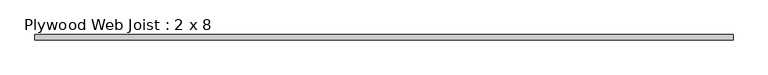
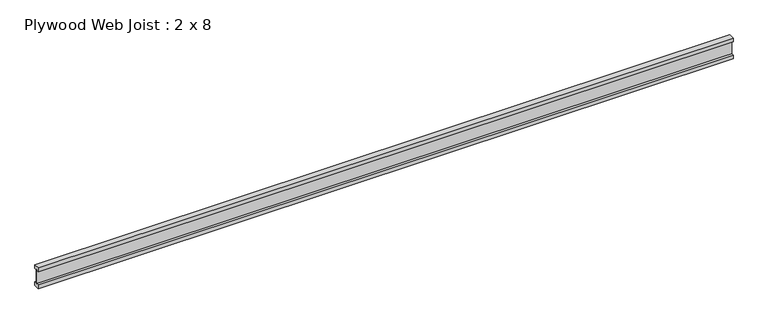
"""IFC4 building model written with IfcOpenShell, lengths in millimetres: beam geometry, Plywood Web Joist : 2 x 8."""

from ifc_helpers import new_model, si_unit, frame, origin, place, context, project, spatial, polyline, outline, extrude, source, transform, mapped, element, save


def plywood_web_joist_2_x_8_156d774c(model_context):
    return source(origin(), model_context, "Body", "SweptSolid", [
        extrude(outline(polyline([(-25.4, 101.6), (25.4, 101.6), (25.4, 63.5), (4.7625, 63.5), (4.7625, 69.85), (-4.7625, 69.85), (-4.7625, 63.5), (-25.4, 63.5), (-25.4, 101.6)])), frame((-3195.5616975, 0.0, 0.0), z_axis=(1.0, 0.0, 0.0), x_axis=(0.0, 1.0, 0.0)), (0.0, 0.0, 1.0), 6391.1233951),
        extrude(outline(polyline([(25.4, -63.5), (25.4, -101.6), (-25.4, -101.6), (-25.4, -63.5), (-4.7625, -63.5), (-4.7625, -69.1160374), (4.7625, -69.1160374), (4.7625, -63.5), (25.4, -63.5)])), frame((-3195.5616975, 0.0, 0.0), z_axis=(1.0, 0.0, 0.0), x_axis=(0.0, 1.0, 0.0)), (0.0, 0.0, 1.0), 6391.1233951),
        extrude(outline(polyline([(3195.5616975, 4.7625), (3195.5616975, -4.7625), (-3195.5616975, -4.7625), (-3195.5616975, 4.7625), (3195.5616975, 4.7625)])), frame((0.0, 0.0, -69.1160374), z_axis=(0.0, 0.0, 1.0), x_axis=(1.0, 0.0, 0.0)), (0.0, 0.0, 1.0), 138.9660374),
    ])


if __name__ == "__main__":
    model = new_model("IFC4")
    model_context = context("Model", 3, world=origin())
    ifc_project = project(units=[si_unit("LENGTHUNIT", "METRE", prefix="MILLI")], contexts=[model_context])
    site = spatial("IfcSite", under=ifc_project)
    building = spatial("IfcBuilding", under=site)
    placement = place(None, origin())
    plywood_web_joist_2_x_8_shape = plywood_web_joist_2_x_8_156d774c(model_context)
    element("IfcBeam", 1, ObjectType="Plywood Web Joist : 2 x 8", at=placement, inside=building, context=model_context, shape_type="MappedRepresentation", body=[
        mapped(plywood_web_joist_2_x_8_shape, transform((0.0, 0.0, 0.0), x_axis=(1.0, 0.0, 0.0), y_axis=(0.0, 1.0, 0.0), z_axis=(0.0, 0.0, 1.0))),
    ])
    save(model, "model.ifc")

# Revit data of these elements
# Type "Plywood Web Joist : 2 x 8"
#   Assembly Code = "B10"
#   Length [instance default] = 5' - 0"
#   b = 0' - 2"
#   d = 0' - 8"
#   Structural Material [instance default] = Softwood, Lumber
# Element 1 (IfcBeam, "Plywood Web Joist : 2 x 8")
#   Materials on its faces: "Softwood, Lumber"
# Materials
#   "Softwood, Lumber": class "Wood", colour RGB 144 113 62, transparency 0, Description = "Pinus Echinata", Cost = 0
